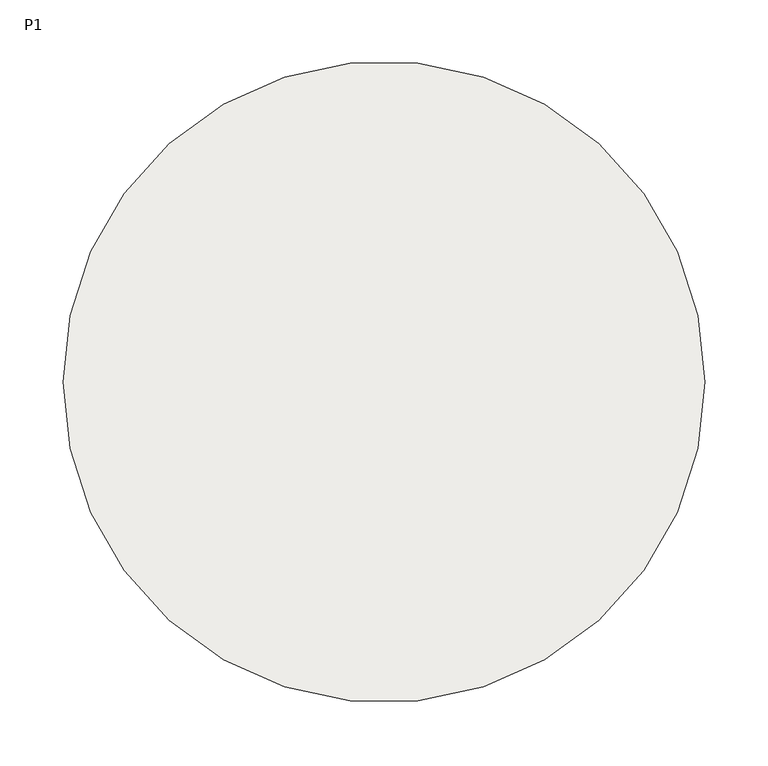
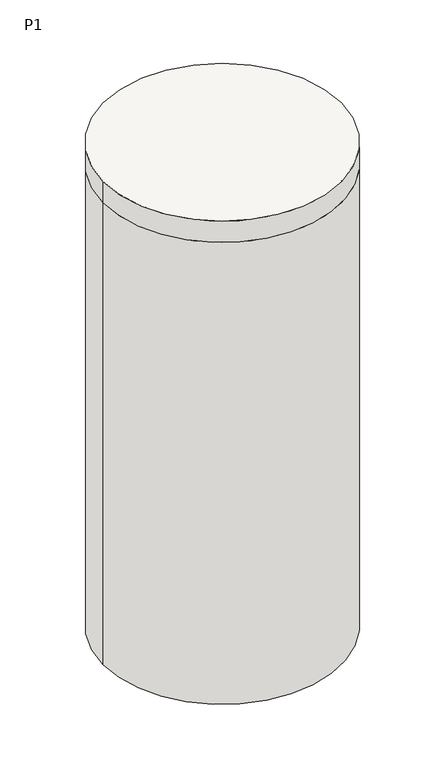
"""IFC4 building model written with IfcOpenShell, lengths in millimetres: slab geometry, Footing-Cylindrical : P1."""

from ifc_helpers import new_model, si_unit, point, frame, origin, origin_with_axes, origin_2d, place, context, project, spatial, circle_curve, trimmed, segment, composite_curve, outline, extrude, source, transform, mapped, element, save


def p1_28f1de1f(model_context):
    return source(origin(), model_context, "Body", "SweptSolid", [
        extrude(outline(composite_curve([segment(trimmed(circle_curve(origin_2d(), 254.0), [point((-254.0, 0.0))], [point((254.0, 0.0))], False, "CARTESIAN"), True, "CONTINUOUS"), segment(trimmed(circle_curve(origin_2d(), 254.0), [point((254.0, 0.0))], [point((-254.0, 0.0))], False, "CARTESIAN"), True, "CONTINUOUS")], self_intersect=False)), origin_with_axes(), (0.0, 0.0, 1.0), 47.625),
        extrude(outline(composite_curve([segment(trimmed(circle_curve(origin_2d(), 254.0), [point((-254.0, 0.0))], [point((254.0, 0.0))], False, "CARTESIAN"), True, "CONTINUOUS"), segment(trimmed(circle_curve(origin_2d(), 254.0), [point((254.0, 0.0))], [point((-254.0, 0.0))], False, "CARTESIAN"), True, "CONTINUOUS")], self_intersect=False)), frame((0.0, 0.0, -1041.4), z_axis=(0.0, 0.0, 1.0), x_axis=(1.0, 0.0, 0.0)), (0.0, 0.0, 1.0), 1041.4),
    ])


if __name__ == "__main__":
    model = new_model("IFC4")
    model_context = context("Model", 3, world=origin())
    ifc_project = project(units=[si_unit("LENGTHUNIT", "METRE", prefix="MILLI")], contexts=[model_context])
    site = spatial("IfcSite", under=ifc_project)
    building = spatial("IfcBuilding", under=site)
    placement = place(None, origin())
    p1_shape = p1_28f1de1f(model_context)
    element("IfcSlab", 1, ObjectType="Footing-Cylindrical : P1", at=placement, inside=building, context=model_context, shape_type="MappedRepresentation", body=[
        mapped(p1_shape, transform((0.0, 0.0, 0.0), x_axis=(1.0, 0.0, 0.0), y_axis=(0.0, 1.0, 0.0), z_axis=(0.0, 0.0, 1.0))),
    ])
    save(model, "model.ifc")

# Revit data of these elements
# Type "Footing-Cylindrical : P1"
#   Assembly Code = "A1010100"
#   Width = 1' - 8"
#   Top Flare Radius = 0' - 10"
#   Radius = 0' - 10"
#   Length = 1' - 8"
#   Foundation Thickness = 3' - 5"
#   Flare Depth = 0' - 1 7/8"
#   Flare Visibility = yes
#   Structural Material = P1: CYLINDRICAL CONCRETE PIER - 20"Øx4'-0" - (4) # 4 VERTICALS - (3) #3 TIES @ 2" OC - REST @ 12" OC
#   Flare Material = 5" CONCRETE SLAB (STAINED/SEALED) WITH WIRE MESH OVER 6 MIL VAPOR BARRIER
# Element 1 (IfcSlab, "Footing-Cylindrical : P1")
#   Materials on its faces: "5\" CONCRETE SLAB (STAINED/SEALED) WITH WIRE MESH OVER 6 MIL VAPOR BARRIER", "P1: CYLINDRICAL CONCRETE PIER - 20\"Øx4'-0\" - (4) # 4 VERTICALS - (3) #3 TIES @ 2\" OC - REST @ 12\" OC"
# Materials
#   "P1: CYLINDRICAL CONCRETE PIER - 20\"Øx4'-0\" - (4) # 4 VERTICALS - (3) #3 TIES @ 2\" OC - REST @ 12\" OC": class "Concrete", colour RGB 164 164 164, transparency 0, Description = "Cast-in-place concrete", Cost = 0
#   "5\" CONCRETE SLAB (STAINED/SEALED) WITH WIRE MESH OVER 6 MIL VAPOR BARRIER": class "Concrete", colour RGB 192 192 192, transparency 0, Description = "Cast-in-place concrete", Cost = 0
